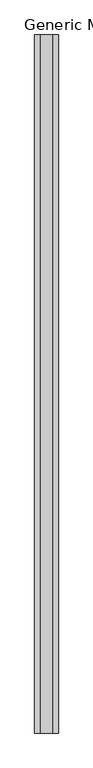
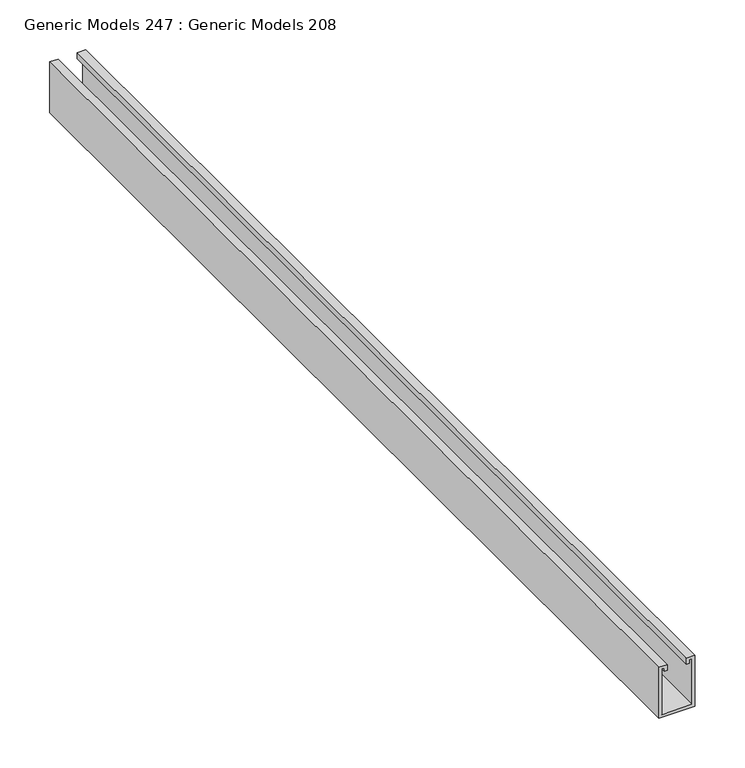
"""IFC4 building model written with IfcOpenShell, lengths in millimetres: proxy geometry, Generic Models 247 : Generic Models 208."""

from ifc_helpers import new_model, si_unit, frame, origin, place, context, project, spatial, polyline, outline, extrude, source, transform, mapped, element, save


def generic_models_247_generic_models_208_75fb8c2a(model_context):
    return source(origin(), model_context, "Body", "SweptSolid", [
        extrude(outline(polyline([(1809.75, 54111.5129445), (1865.3125, 54111.5129445), (1865.3125, 54114.6879445), (1861.34375, 54114.6879445), (1861.34375, 54117.8629445), (1868.4875, 54117.8629445), (1868.4875, 54108.3379445), (1806.575, 54108.3379445), (1806.575, 54149.6129445), (1868.4875, 54149.6129445), (1868.4875, 54140.0879445), (1861.34375, 54140.0879445), (1861.34375, 54143.2629445), (1865.3125, 54143.2629445), (1865.3125, 54146.4379445), (1809.75, 54146.4379445), (1809.75, 54111.5129445)])), frame((0.0, -228.7033818, 0.0), z_axis=(0.0, 1.0, 0.0), x_axis=(0.0, 0.0, 1.0)), (0.0, 0.0, 1.0), 1219.2),
    ])


if __name__ == "__main__":
    model = new_model("IFC4")
    model_context = context("Model", 3, world=origin())
    ifc_project = project(units=[si_unit("LENGTHUNIT", "METRE", prefix="MILLI")], contexts=[model_context])
    site = spatial("IfcSite", under=ifc_project)
    building = spatial("IfcBuilding", under=site)
    placement = place(None, origin())
    generic_models_247_generic_models_208_shape = generic_models_247_generic_models_208_75fb8c2a(model_context)
    element("IfcBuildingElementProxy", 1, Name="Generic Models 247 : Generic Models 208", ObjectType="Generic Models 247 : Generic Models 208", at=placement, inside=building, context=model_context, shape_type="MappedRepresentation", body=[
        mapped(generic_models_247_generic_models_208_shape, transform((0.0, 0.0, 0.0), x_axis=(1.0, 0.0, 0.0), y_axis=(0.0, 1.0, 0.0), z_axis=(0.0, 0.0, 1.0))),
    ])
    save(model, "model.ifc")
